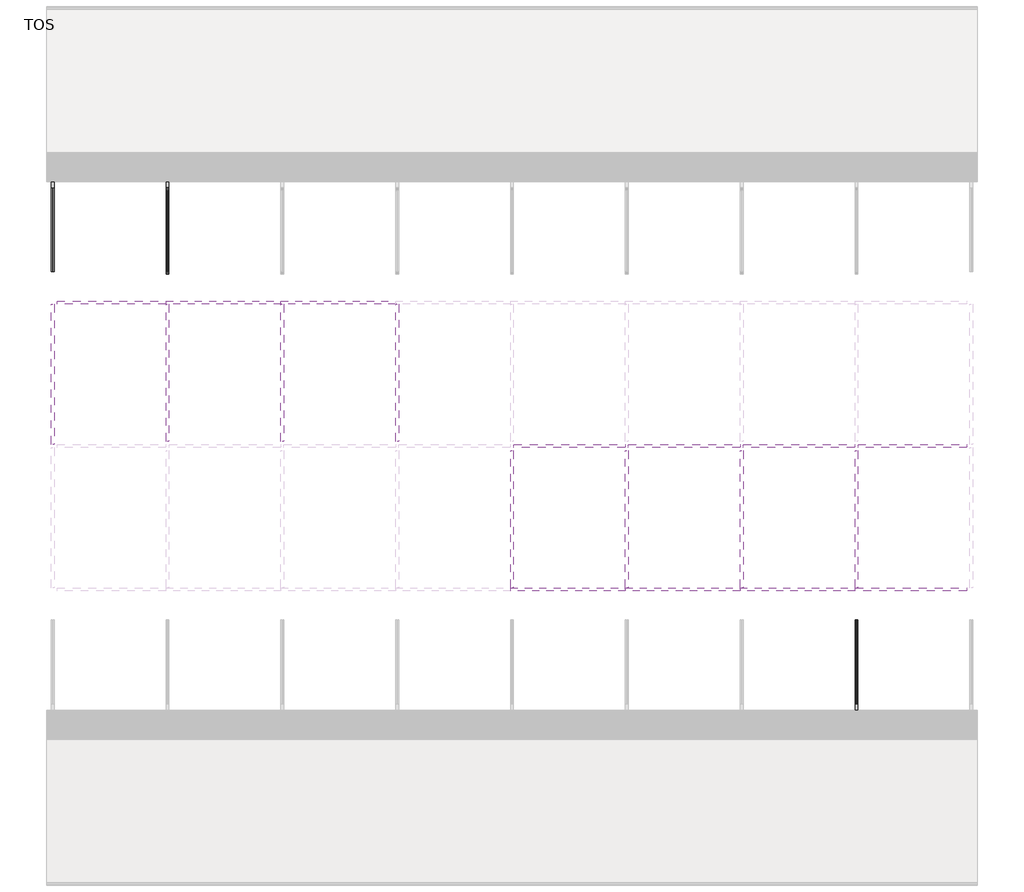
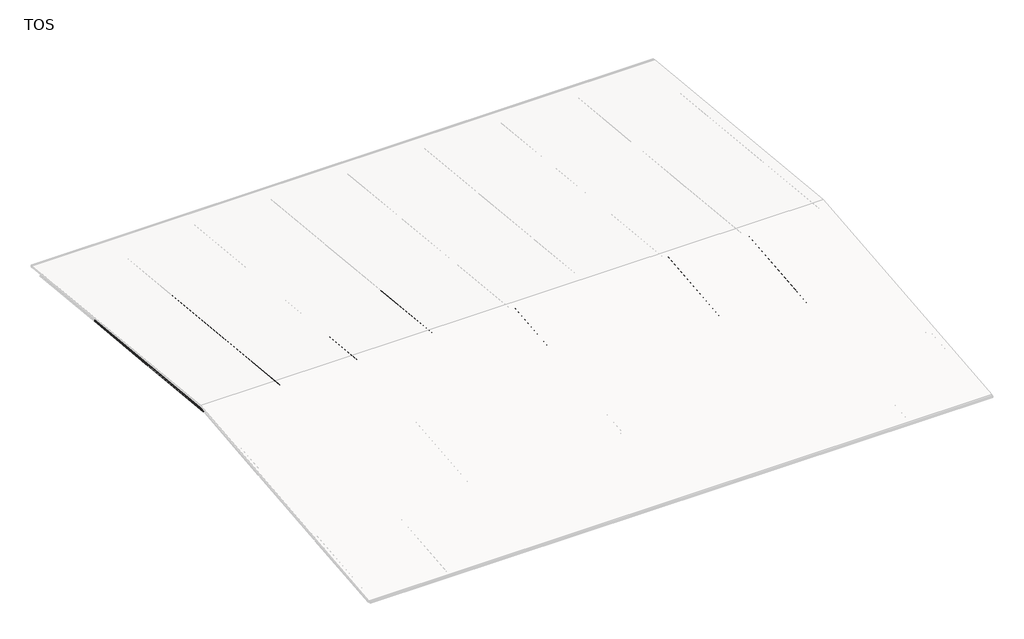
# One storey, part 3 of 5: 22 beams.
"""IFC4 building model written with IfcOpenShell, lengths in millimetres."""

from ifc_helpers import new_model, si_unit, point, frame, frame_2d, origin, place, context, project, spatial, polyline, circle_curve, trimmed, segment, composite_curve, outline, extrude, element, save

model = new_model("IFC4")

# Units and contexts
model_context = context("Model", 3, world=origin())
ifc_project = project(units=[si_unit("LENGTHUNIT", "METRE", prefix="MILLI")], contexts=[model_context])

# Site, building, storey
site = spatial("IfcSite", under=ifc_project)
building = spatial("IfcBuilding", under=site)
storey = spatial("IfcBuildingStorey", under=building, Name="TOS", Elevation=9299.9618634)

# Beams
placement = place(None, origin())
element("IfcBeam", 1, ObjectType="0912_Steel Framing_H-KSD3502 : H_SB_ASB_H-600x200x11x17", at=placement, inside=storey, context=model_context, shape_type="SweptSolid", body=[
    extrude(outline(composite_curve([segment(polyline([(20599.5208589, 10716.9618634), (20599.5208589, 10699.9618634), (20399.5208589, 10699.9618634), (20399.5208589, 10716.9618634), (20472.0208589, 10716.9618634)]), True, "CONTINUOUS"), segment(trimmed(circle_curve(frame_2d((20472.0208589, 10738.9618634)), 22.0), [point((20472.0208589, 10716.9618634))], [point((20494.0208589, 10738.9618634))], True, "CARTESIAN"), True, "CONTINUOUS"), segment(polyline([(20494.0208589, 10738.9618634), (20494.0208589, 11260.9618634)]), True, "CONTINUOUS"), segment(trimmed(circle_curve(frame_2d((20472.0208589, 11260.9618634)), 22.0), [point((20494.0208589, 11260.9618634))], [point((20472.0208589, 11282.9618634))], True, "CARTESIAN"), True, "CONTINUOUS"), segment(polyline([(20472.0208589, 11282.9618634), (20399.5208589, 11282.9618634), (20399.5208589, 11299.9618634), (20599.5208589, 11299.9618634), (20599.5208589, 11282.9618634), (20527.0208589, 11282.9618634)]), True, "CONTINUOUS"), segment(trimmed(circle_curve(frame_2d((20527.0208589, 11260.9618634)), 22.0), [point((20527.0208589, 11282.9618634))], [point((20505.0208589, 11260.9618634))], True, "CARTESIAN"), True, "CONTINUOUS"), segment(polyline([(20505.0208589, 11260.9618634), (20505.0208589, 10738.9618634)]), True, "CONTINUOUS"), segment(trimmed(circle_curve(frame_2d((20527.0208589, 10738.9618634)), 22.0), [point((20505.0208589, 10738.9618634))], [point((20527.0208589, 10716.9618634))], True, "CARTESIAN"), True, "CONTINUOUS"), segment(polyline([(20527.0208589, 10716.9618634), (20599.5208589, 10716.9618634)]), True, "CONTINUOUS")], self_intersect=False)), frame((31900.0, 0.0, 0.0), z_axis=(1.0, 0.0, 0.0), x_axis=(0.0, 1.0, 0.0)), (0.0, 0.0, 1.0), 7987.3),
])
element("IfcBeam", 2, ObjectType="0912_Steel Framing_H-KSD3502 : H_SB_ASB_H-600x200x11x17", at=placement, inside=storey, context=model_context, shape_type="SweptSolid", body=[
    extrude(outline(composite_curve([segment(polyline([(20599.5208589, 10716.9618634), (20599.5208589, 10699.9618634), (20399.5208589, 10699.9618634), (20399.5208589, 10716.9618634), (20472.0208589, 10716.9618634)]), True, "CONTINUOUS"), segment(trimmed(circle_curve(frame_2d((20472.0208589, 10738.9618634)), 22.0), [point((20472.0208589, 10716.9618634))], [point((20494.0208589, 10738.9618634))], True, "CARTESIAN"), True, "CONTINUOUS"), segment(polyline([(20494.0208589, 10738.9618634), (20494.0208589, 11260.9618634)]), True, "CONTINUOUS"), segment(trimmed(circle_curve(frame_2d((20472.0208589, 11260.9618634)), 22.0), [point((20494.0208589, 11260.9618634))], [point((20472.0208589, 11282.9618634))], True, "CARTESIAN"), True, "CONTINUOUS"), segment(polyline([(20472.0208589, 11282.9618634), (20399.5208589, 11282.9618634), (20399.5208589, 11299.9618634), (20599.5208589, 11299.9618634), (20599.5208589, 11282.9618634), (20527.0208589, 11282.9618634)]), True, "CONTINUOUS"), segment(trimmed(circle_curve(frame_2d((20527.0208589, 11260.9618634)), 22.0), [point((20527.0208589, 11282.9618634))], [point((20505.0208589, 11260.9618634))], True, "CARTESIAN"), True, "CONTINUOUS"), segment(polyline([(20505.0208589, 11260.9618634), (20505.0208589, 10738.9618634)]), True, "CONTINUOUS"), segment(trimmed(circle_curve(frame_2d((20527.0208589, 10738.9618634)), 22.0), [point((20505.0208589, 10738.9618634))], [point((20527.0208589, 10716.9618634))], True, "CARTESIAN"), True, "CONTINUOUS"), segment(polyline([(20527.0208589, 10716.9618634), (20599.5208589, 10716.9618634)]), True, "CONTINUOUS")], self_intersect=False)), frame((39900.0, 0.0, 0.0), z_axis=(1.0, 0.0, 0.0), x_axis=(0.0, 1.0, 0.0)), (0.0, 0.0, 1.0), 7987.3),
])
element("IfcBeam", 3, ObjectType="0912_Steel Framing_H-KSD3502 : H_SB_ASB_H-600x200x11x17", at=placement, inside=storey, context=model_context, shape_type="SweptSolid", body=[
    extrude(outline(composite_curve([segment(polyline([(20599.5208589, 10716.9618634), (20599.5208589, 10699.9618634), (20399.5208589, 10699.9618634), (20399.5208589, 10716.9618634), (20472.0208589, 10716.9618634)]), True, "CONTINUOUS"), segment(trimmed(circle_curve(frame_2d((20472.0208589, 10738.9618634)), 22.0), [point((20472.0208589, 10716.9618634))], [point((20494.0208589, 10738.9618634))], True, "CARTESIAN"), True, "CONTINUOUS"), segment(polyline([(20494.0208589, 10738.9618634), (20494.0208589, 11260.9618634)]), True, "CONTINUOUS"), segment(trimmed(circle_curve(frame_2d((20472.0208589, 11260.9618634)), 22.0), [point((20494.0208589, 11260.9618634))], [point((20472.0208589, 11282.9618634))], True, "CARTESIAN"), True, "CONTINUOUS"), segment(polyline([(20472.0208589, 11282.9618634), (20399.5208589, 11282.9618634), (20399.5208589, 11299.9618634), (20599.5208589, 11299.9618634), (20599.5208589, 11282.9618634), (20527.0208589, 11282.9618634)]), True, "CONTINUOUS"), segment(trimmed(circle_curve(frame_2d((20527.0208589, 11260.9618634)), 22.0), [point((20527.0208589, 11282.9618634))], [point((20505.0208589, 11260.9618634))], True, "CARTESIAN"), True, "CONTINUOUS"), segment(polyline([(20505.0208589, 11260.9618634), (20505.0208589, 10738.9618634)]), True, "CONTINUOUS"), segment(trimmed(circle_curve(frame_2d((20527.0208589, 10738.9618634)), 22.0), [point((20505.0208589, 10738.9618634))], [point((20527.0208589, 10716.9618634))], True, "CARTESIAN"), True, "CONTINUOUS"), segment(polyline([(20527.0208589, 10716.9618634), (20599.5208589, 10716.9618634)]), True, "CONTINUOUS")], self_intersect=False)), frame((47900.0, 0.0, 0.0), z_axis=(1.0, 0.0, 0.0), x_axis=(0.0, 1.0, 0.0)), (0.0, 0.0, 1.0), 7987.3),
])
element("IfcBeam", 4, ObjectType="0912_Steel Framing_H-KSD3502 : H_SB_ASB_H-600x200x11x17", at=placement, inside=storey, context=model_context, shape_type="SweptSolid", body=[
    extrude(outline(composite_curve([segment(polyline([(20599.5208589, 10716.9618634), (20599.5208589, 10699.9618634), (20399.5208589, 10699.9618634), (20399.5208589, 10716.9618634), (20472.0208589, 10716.9618634)]), True, "CONTINUOUS"), segment(trimmed(circle_curve(frame_2d((20472.0208589, 10738.9618634)), 22.0), [point((20472.0208589, 10716.9618634))], [point((20494.0208589, 10738.9618634))], True, "CARTESIAN"), True, "CONTINUOUS"), segment(polyline([(20494.0208589, 10738.9618634), (20494.0208589, 11260.9618634)]), True, "CONTINUOUS"), segment(trimmed(circle_curve(frame_2d((20472.0208589, 11260.9618634)), 22.0), [point((20494.0208589, 11260.9618634))], [point((20472.0208589, 11282.9618634))], True, "CARTESIAN"), True, "CONTINUOUS"), segment(polyline([(20472.0208589, 11282.9618634), (20399.5208589, 11282.9618634), (20399.5208589, 11299.9618634), (20599.5208589, 11299.9618634), (20599.5208589, 11282.9618634), (20527.0208589, 11282.9618634)]), True, "CONTINUOUS"), segment(trimmed(circle_curve(frame_2d((20527.0208589, 11260.9618634)), 22.0), [point((20527.0208589, 11282.9618634))], [point((20505.0208589, 11260.9618634))], True, "CARTESIAN"), True, "CONTINUOUS"), segment(polyline([(20505.0208589, 11260.9618634), (20505.0208589, 10738.9618634)]), True, "CONTINUOUS"), segment(trimmed(circle_curve(frame_2d((20527.0208589, 10738.9618634)), 22.0), [point((20505.0208589, 10738.9618634))], [point((20527.0208589, 10716.9618634))], True, "CARTESIAN"), True, "CONTINUOUS"), segment(polyline([(20527.0208589, 10716.9618634), (20599.5208589, 10716.9618634)]), True, "CONTINUOUS")], self_intersect=False)), frame((55900.0, 0.0, 0.0), z_axis=(1.0, 0.0, 0.0), x_axis=(0.0, 1.0, 0.0)), (0.0, 0.0, 1.0), 7781.3),
])
element("IfcBeam", 5, ObjectType="0912_Steel Framing_H-KSD3502 : H_SB_ASB_H-600x200x11x17", at=placement, inside=storey, context=model_context, shape_type="SweptSolid", body=[
    extrude(outline(composite_curve([segment(polyline([(30599.5208589, 11716.9618634), (30599.5208589, 11699.9618634), (30399.5208589, 11699.9618634), (30399.5208589, 11716.9618634), (30472.0208589, 11716.9618634)]), True, "CONTINUOUS"), segment(trimmed(circle_curve(frame_2d((30472.0208589, 11738.9618634)), 22.0), [point((30472.0208589, 11716.9618634))], [point((30494.0208589, 11738.9618634))], True, "CARTESIAN"), True, "CONTINUOUS"), segment(polyline([(30494.0208589, 11738.9618634), (30494.0208589, 12260.9618634)]), True, "CONTINUOUS"), segment(trimmed(circle_curve(frame_2d((30472.0208589, 12260.9618634)), 22.0), [point((30494.0208589, 12260.9618634))], [point((30472.0208589, 12282.9618634))], True, "CARTESIAN"), True, "CONTINUOUS"), segment(polyline([(30472.0208589, 12282.9618634), (30399.5208589, 12282.9618634), (30399.5208589, 12299.9618634), (30599.5208589, 12299.9618634), (30599.5208589, 12282.9618634), (30527.0208589, 12282.9618634)]), True, "CONTINUOUS"), segment(trimmed(circle_curve(frame_2d((30527.0208589, 12260.9618634)), 22.0), [point((30527.0208589, 12282.9618634))], [point((30505.0208589, 12260.9618634))], True, "CARTESIAN"), True, "CONTINUOUS"), segment(polyline([(30505.0208589, 12260.9618634), (30505.0208589, 11738.9618634)]), True, "CONTINUOUS"), segment(trimmed(circle_curve(frame_2d((30527.0208589, 11738.9618634)), 22.0), [point((30505.0208589, 11738.9618634))], [point((30527.0208589, 11716.9618634))], True, "CARTESIAN"), True, "CONTINUOUS"), segment(polyline([(30527.0208589, 11716.9618634), (30599.5208589, 11716.9618634)]), True, "CONTINUOUS")], self_intersect=False)), frame((32113.7, 0.0, 0.0), z_axis=(1.0, 0.0, 0.0), x_axis=(0.0, 1.0, 0.0)), (0.0, 0.0, 1.0), 7772.6),
])
element("IfcBeam", 6, ObjectType="0912_Steel Framing_H-KSD3502 : H_SB_ASB_H-600x200x11x17", at=placement, inside=storey, context=model_context, shape_type="SweptSolid", body=[
    extrude(outline(composite_curve([segment(polyline([(30599.5208589, 11716.9618634), (30599.5208589, 11699.9618634), (30399.5208589, 11699.9618634), (30399.5208589, 11716.9618634), (30472.0208589, 11716.9618634)]), True, "CONTINUOUS"), segment(trimmed(circle_curve(frame_2d((30472.0208589, 11738.9618634)), 22.0), [point((30472.0208589, 11716.9618634))], [point((30494.0208589, 11738.9618634))], True, "CARTESIAN"), True, "CONTINUOUS"), segment(polyline([(30494.0208589, 11738.9618634), (30494.0208589, 12260.9618634)]), True, "CONTINUOUS"), segment(trimmed(circle_curve(frame_2d((30472.0208589, 12260.9618634)), 22.0), [point((30494.0208589, 12260.9618634))], [point((30472.0208589, 12282.9618634))], True, "CARTESIAN"), True, "CONTINUOUS"), segment(polyline([(30472.0208589, 12282.9618634), (30399.5208589, 12282.9618634), (30399.5208589, 12299.9618634), (30599.5208589, 12299.9618634), (30599.5208589, 12282.9618634), (30527.0208589, 12282.9618634)]), True, "CONTINUOUS"), segment(trimmed(circle_curve(frame_2d((30527.0208589, 12260.9618634)), 22.0), [point((30527.0208589, 12282.9618634))], [point((30505.0208589, 12260.9618634))], True, "CARTESIAN"), True, "CONTINUOUS"), segment(polyline([(30505.0208589, 12260.9618634), (30505.0208589, 11738.9618634)]), True, "CONTINUOUS"), segment(trimmed(circle_curve(frame_2d((30527.0208589, 11738.9618634)), 22.0), [point((30505.0208589, 11738.9618634))], [point((30527.0208589, 11716.9618634))], True, "CARTESIAN"), True, "CONTINUOUS"), segment(polyline([(30527.0208589, 11716.9618634), (30599.5208589, 11716.9618634)]), True, "CONTINUOUS")], self_intersect=False)), frame((40113.7, 0.0, 0.0), z_axis=(1.0, 0.0, 0.0), x_axis=(0.0, 1.0, 0.0)), (0.0, 0.0, 1.0), 7772.6),
])
element("IfcBeam", 7, ObjectType="0912_Steel Framing_H-KSD3502 : H_SB_ASB_H-600x200x11x17", at=placement, inside=storey, context=model_context, shape_type="SweptSolid", body=[
    extrude(outline(composite_curve([segment(polyline([(30599.5208589, 11716.9618634), (30599.5208589, 11699.9618634), (30399.5208589, 11699.9618634), (30399.5208589, 11716.9618634), (30472.0208589, 11716.9618634)]), True, "CONTINUOUS"), segment(trimmed(circle_curve(frame_2d((30472.0208589, 11738.9618634)), 22.0), [point((30472.0208589, 11716.9618634))], [point((30494.0208589, 11738.9618634))], True, "CARTESIAN"), True, "CONTINUOUS"), segment(polyline([(30494.0208589, 11738.9618634), (30494.0208589, 12260.9618634)]), True, "CONTINUOUS"), segment(trimmed(circle_curve(frame_2d((30472.0208589, 12260.9618634)), 22.0), [point((30494.0208589, 12260.9618634))], [point((30472.0208589, 12282.9618634))], True, "CARTESIAN"), True, "CONTINUOUS"), segment(polyline([(30472.0208589, 12282.9618634), (30399.5208589, 12282.9618634), (30399.5208589, 12299.9618634), (30599.5208589, 12299.9618634), (30599.5208589, 12282.9618634), (30527.0208589, 12282.9618634)]), True, "CONTINUOUS"), segment(trimmed(circle_curve(frame_2d((30527.0208589, 12260.9618634)), 22.0), [point((30527.0208589, 12282.9618634))], [point((30505.0208589, 12260.9618634))], True, "CARTESIAN"), True, "CONTINUOUS"), segment(polyline([(30505.0208589, 12260.9618634), (30505.0208589, 11738.9618634)]), True, "CONTINUOUS"), segment(trimmed(circle_curve(frame_2d((30527.0208589, 11738.9618634)), 22.0), [point((30505.0208589, 11738.9618634))], [point((30527.0208589, 11716.9618634))], True, "CARTESIAN"), True, "CONTINUOUS"), segment(polyline([(30527.0208589, 11716.9618634), (30599.5208589, 11716.9618634)]), True, "CONTINUOUS")], self_intersect=False)), frame((48113.7, 0.0, 0.0), z_axis=(1.0, 0.0, 0.0), x_axis=(0.0, 1.0, 0.0)), (0.0, 0.0, 1.0), 7772.6),
])
element("IfcBeam", 8, ObjectType="0912_Steel Framing_H-KSD3502 : H_SB_ASB_H-600x200x11x17", at=placement, inside=storey, context=model_context, shape_type="SweptSolid", body=[
    extrude(outline(composite_curve([segment(polyline([(30599.5208589, 11716.9618634), (30599.5208589, 11699.9618634), (30399.5208589, 11699.9618634), (30399.5208589, 11716.9618634), (30472.0208589, 11716.9618634)]), True, "CONTINUOUS"), segment(trimmed(circle_curve(frame_2d((30472.0208589, 11738.9618634)), 22.0), [point((30472.0208589, 11716.9618634))], [point((30494.0208589, 11738.9618634))], True, "CARTESIAN"), True, "CONTINUOUS"), segment(polyline([(30494.0208589, 11738.9618634), (30494.0208589, 12260.9618634)]), True, "CONTINUOUS"), segment(trimmed(circle_curve(frame_2d((30472.0208589, 12260.9618634)), 22.0), [point((30494.0208589, 12260.9618634))], [point((30472.0208589, 12282.9618634))], True, "CARTESIAN"), True, "CONTINUOUS"), segment(polyline([(30472.0208589, 12282.9618634), (30399.5208589, 12282.9618634), (30399.5208589, 12299.9618634), (30599.5208589, 12299.9618634), (30599.5208589, 12282.9618634), (30527.0208589, 12282.9618634)]), True, "CONTINUOUS"), segment(trimmed(circle_curve(frame_2d((30527.0208589, 12260.9618634)), 22.0), [point((30527.0208589, 12282.9618634))], [point((30505.0208589, 12260.9618634))], True, "CARTESIAN"), True, "CONTINUOUS"), segment(polyline([(30505.0208589, 12260.9618634), (30505.0208589, 11738.9618634)]), True, "CONTINUOUS"), segment(trimmed(circle_curve(frame_2d((30527.0208589, 11738.9618634)), 22.0), [point((30505.0208589, 11738.9618634))], [point((30527.0208589, 11716.9618634))], True, "CARTESIAN"), True, "CONTINUOUS"), segment(polyline([(30527.0208589, 11716.9618634), (30599.5208589, 11716.9618634)]), True, "CONTINUOUS")], self_intersect=False)), frame((56113.7, 0.0, 0.0), z_axis=(1.0, 0.0, 0.0), x_axis=(0.0, 1.0, 0.0)), (0.0, 0.0, 1.0), 7567.6),
])
element("IfcBeam", 9, ObjectType="0912_Steel Framing_H-KSD3502 : H_SB_ASB_H-600x200x11x17", at=placement, inside=storey, context=model_context, shape_type="SweptSolid", body=[
    extrude(outline(composite_curve([segment(polyline([(40599.5208589, 10716.9618634), (40599.5208589, 10699.9618634), (40399.5208589, 10699.9618634), (40399.5208589, 10716.9618634), (40472.0208589, 10716.9618634)]), True, "CONTINUOUS"), segment(trimmed(circle_curve(frame_2d((40472.0208589, 10738.9618634)), 22.0), [point((40472.0208589, 10716.9618634))], [point((40494.0208589, 10738.9618634))], True, "CARTESIAN"), True, "CONTINUOUS"), segment(polyline([(40494.0208589, 10738.9618634), (40494.0208589, 11260.9618634)]), True, "CONTINUOUS"), segment(trimmed(circle_curve(frame_2d((40472.0208589, 11260.9618634)), 22.0), [point((40494.0208589, 11260.9618634))], [point((40472.0208589, 11282.9618634))], True, "CARTESIAN"), True, "CONTINUOUS"), segment(polyline([(40472.0208589, 11282.9618634), (40399.5208589, 11282.9618634), (40399.5208589, 11299.9618634), (40599.5208589, 11299.9618634), (40599.5208589, 11282.9618634), (40527.0208589, 11282.9618634)]), True, "CONTINUOUS"), segment(trimmed(circle_curve(frame_2d((40527.0208589, 11260.9618634)), 22.0), [point((40527.0208589, 11282.9618634))], [point((40505.0208589, 11260.9618634))], True, "CARTESIAN"), True, "CONTINUOUS"), segment(polyline([(40505.0208589, 11260.9618634), (40505.0208589, 10738.9618634)]), True, "CONTINUOUS"), segment(trimmed(circle_curve(frame_2d((40527.0208589, 10738.9618634)), 22.0), [point((40505.0208589, 10738.9618634))], [point((40527.0208589, 10716.9618634))], True, "CARTESIAN"), True, "CONTINUOUS"), segment(polyline([(40527.0208589, 10716.9618634), (40599.5208589, 10716.9618634)]), True, "CONTINUOUS")], self_intersect=False)), frame((318.7, 0.0, 0.0), z_axis=(1.0, 0.0, 0.0), x_axis=(0.0, 1.0, 0.0)), (0.0, 0.0, 1.0), 7568.6),
])
element("IfcBeam", 10, ObjectType="0912_Steel Framing_H-KSD3502 : H_SB_ASB_H-600x200x11x17", at=placement, inside=storey, context=model_context, shape_type="SweptSolid", body=[
    extrude(outline(composite_curve([segment(polyline([(40599.5208589, 10716.9618634), (40599.5208589, 10699.9618634), (40399.5208589, 10699.9618634), (40399.5208589, 10716.9618634), (40472.0208589, 10716.9618634)]), True, "CONTINUOUS"), segment(trimmed(circle_curve(frame_2d((40472.0208589, 10738.9618634)), 22.0), [point((40472.0208589, 10716.9618634))], [point((40494.0208589, 10738.9618634))], True, "CARTESIAN"), True, "CONTINUOUS"), segment(polyline([(40494.0208589, 10738.9618634), (40494.0208589, 11260.9618634)]), True, "CONTINUOUS"), segment(trimmed(circle_curve(frame_2d((40472.0208589, 11260.9618634)), 22.0), [point((40494.0208589, 11260.9618634))], [point((40472.0208589, 11282.9618634))], True, "CARTESIAN"), True, "CONTINUOUS"), segment(polyline([(40472.0208589, 11282.9618634), (40399.5208589, 11282.9618634), (40399.5208589, 11299.9618634), (40599.5208589, 11299.9618634), (40599.5208589, 11282.9618634), (40527.0208589, 11282.9618634)]), True, "CONTINUOUS"), segment(trimmed(circle_curve(frame_2d((40527.0208589, 11260.9618634)), 22.0), [point((40527.0208589, 11282.9618634))], [point((40505.0208589, 11260.9618634))], True, "CARTESIAN"), True, "CONTINUOUS"), segment(polyline([(40505.0208589, 11260.9618634), (40505.0208589, 10738.9618634)]), True, "CONTINUOUS"), segment(trimmed(circle_curve(frame_2d((40527.0208589, 10738.9618634)), 22.0), [point((40505.0208589, 10738.9618634))], [point((40527.0208589, 10716.9618634))], True, "CARTESIAN"), True, "CONTINUOUS"), segment(polyline([(40527.0208589, 10716.9618634), (40599.5208589, 10716.9618634)]), True, "CONTINUOUS")], self_intersect=False)), frame((7900.0, 0.0, 0.0), z_axis=(1.0, 0.0, 0.0), x_axis=(0.0, 1.0, 0.0)), (0.0, 0.0, 1.0), 7987.3),
])
element("IfcBeam", 11, ObjectType="0912_Steel Framing_H-KSD3502 : H_SB_ASB_H-600x200x11x17", at=placement, inside=storey, context=model_context, shape_type="SweptSolid", body=[
    extrude(outline(composite_curve([segment(polyline([(40599.5208589, 10716.9618634), (40599.5208589, 10699.9618634), (40399.5208589, 10699.9618634), (40399.5208589, 10716.9618634), (40472.0208589, 10716.9618634)]), True, "CONTINUOUS"), segment(trimmed(circle_curve(frame_2d((40472.0208589, 10738.9618634)), 22.0), [point((40472.0208589, 10716.9618634))], [point((40494.0208589, 10738.9618634))], True, "CARTESIAN"), True, "CONTINUOUS"), segment(polyline([(40494.0208589, 10738.9618634), (40494.0208589, 11260.9618634)]), True, "CONTINUOUS"), segment(trimmed(circle_curve(frame_2d((40472.0208589, 11260.9618634)), 22.0), [point((40494.0208589, 11260.9618634))], [point((40472.0208589, 11282.9618634))], True, "CARTESIAN"), True, "CONTINUOUS"), segment(polyline([(40472.0208589, 11282.9618634), (40399.5208589, 11282.9618634), (40399.5208589, 11299.9618634), (40599.5208589, 11299.9618634), (40599.5208589, 11282.9618634), (40527.0208589, 11282.9618634)]), True, "CONTINUOUS"), segment(trimmed(circle_curve(frame_2d((40527.0208589, 11260.9618634)), 22.0), [point((40527.0208589, 11282.9618634))], [point((40505.0208589, 11260.9618634))], True, "CARTESIAN"), True, "CONTINUOUS"), segment(polyline([(40505.0208589, 11260.9618634), (40505.0208589, 10738.9618634)]), True, "CONTINUOUS"), segment(trimmed(circle_curve(frame_2d((40527.0208589, 10738.9618634)), 22.0), [point((40505.0208589, 10738.9618634))], [point((40527.0208589, 10716.9618634))], True, "CARTESIAN"), True, "CONTINUOUS"), segment(polyline([(40527.0208589, 10716.9618634), (40599.5208589, 10716.9618634)]), True, "CONTINUOUS")], self_intersect=False)), frame((15900.0, 0.0, 0.0), z_axis=(1.0, 0.0, 0.0), x_axis=(0.0, 1.0, 0.0)), (0.0, 0.0, 1.0), 7987.3),
])
element("IfcBeam", 12, ObjectType="0912_Steel Framing_H-KSD3502 : H_SB_ASB_H-600x200x11x17", at=placement, inside=storey, context=model_context, shape_type="SweptSolid", body=[
    extrude(outline(composite_curve([segment(polyline([(-283.0, 100.0), (-283.0, 27.5)]), True, "CONTINUOUS"), segment(trimmed(circle_curve(frame_2d((-261.0, 27.5)), 22.0), [point((-283.0, 27.5))], [point((-261.0, 5.5))], True, "CARTESIAN"), True, "CONTINUOUS"), segment(polyline([(-261.0, 5.5), (261.0, 5.5)]), True, "CONTINUOUS"), segment(trimmed(circle_curve(frame_2d((261.0, 27.5)), 22.0), [point((261.0, 5.5))], [point((283.0000001, 27.5))], True, "CARTESIAN"), True, "CONTINUOUS"), segment(polyline([(283.0000001, 27.5), (283.0000001, 100.0), (300.0, 100.0), (300.0, -100.0), (283.0000001, -100.0), (283.0000001, -27.5)]), True, "CONTINUOUS"), segment(trimmed(circle_curve(frame_2d((261.0, -27.5)), 22.0), [point((283.0000001, -27.5))], [point((261.0, -5.5))], True, "CARTESIAN"), True, "CONTINUOUS"), segment(polyline([(261.0, -5.5), (-261.0, -5.5)]), True, "CONTINUOUS"), segment(trimmed(circle_curve(frame_2d((-261.0, -27.5)), 22.0), [point((-261.0, -5.5))], [point((-283.0, -27.5))], True, "CARTESIAN"), True, "CONTINUOUS"), segment(polyline([(-283.0, -27.5), (-283.0, -100.0), (-299.9999999, -100.0), (-299.9999999, 100.0), (-283.0, 100.0)]), True, "CONTINUOUS")], self_intersect=False)), frame((0.0, 40357.0327709, 11012.7144035), z_axis=(0.0, -0.9950371902099892, 0.09950371902099892), x_axis=(0.0, 0.09950371902099892, 0.9950371902099892)), (0.0, 0.0, 1.0), 9762.4731211),
])
element("IfcBeam", 13, ObjectType="0912_Steel Framing_H-KSD3502 : H_SB_ASB_H-600x200x11x17", at=placement, inside=storey, context=model_context, shape_type="SweptSolid", body=[
    extrude(outline(composite_curve([segment(polyline([(-283.0, 100.0), (-283.0, 27.5)]), True, "CONTINUOUS"), segment(trimmed(circle_curve(frame_2d((-261.0, 27.5)), 22.0), [point((-283.0, 27.5))], [point((-261.0, 5.5))], True, "CARTESIAN"), True, "CONTINUOUS"), segment(polyline([(-261.0, 5.5), (261.0, 5.5)]), True, "CONTINUOUS"), segment(trimmed(circle_curve(frame_2d((261.0, 27.5)), 22.0), [point((261.0, 5.5))], [point((283.0000001, 27.5))], True, "CARTESIAN"), True, "CONTINUOUS"), segment(polyline([(283.0000001, 27.5), (283.0000001, 100.0), (300.0, 100.0), (300.0, -100.0), (283.0000001, -100.0), (283.0000001, -27.5)]), True, "CONTINUOUS"), segment(trimmed(circle_curve(frame_2d((261.0, -27.5)), 22.0), [point((283.0000001, -27.5))], [point((261.0, -5.5))], True, "CARTESIAN"), True, "CONTINUOUS"), segment(polyline([(261.0, -5.5), (-261.0, -5.5)]), True, "CONTINUOUS"), segment(trimmed(circle_curve(frame_2d((-261.0, -27.5)), 22.0), [point((-261.0, -5.5))], [point((-283.0, -27.5))], True, "CARTESIAN"), True, "CONTINUOUS"), segment(polyline([(-283.0, -27.5), (-283.0, -100.0), (-299.9999999, -100.0), (-299.9999999, 100.0), (-283.0, 100.0)]), True, "CONTINUOUS")], self_intersect=False)), frame((0.0, 50357.0327709, 10012.7144035), z_axis=(0.0, -0.9950371902099892, 0.09950371902099896), x_axis=(0.0, 0.09950371902099896, 0.9950371902099892)), (0.0, 0.0, 1.0), 9762.4731211),
])
element("IfcBeam", 14, ObjectType="0912_Steel Framing_H-KSD3502 : H_SB_ASB_H-600x200x11x17", at=placement, inside=storey, context=model_context, shape_type="SweptSolid", body=[
    extrude(outline(composite_curve([segment(polyline([(-283.0, 100.0), (-283.0, 27.5)]), True, "CONTINUOUS"), segment(trimmed(circle_curve(frame_2d((-261.0, 27.5)), 22.0), [point((-283.0, 27.5))], [point((-261.0, 5.5))], True, "CARTESIAN"), True, "CONTINUOUS"), segment(polyline([(-261.0, 5.5), (261.0, 5.5)]), True, "CONTINUOUS"), segment(trimmed(circle_curve(frame_2d((261.0, 27.5)), 22.0), [point((261.0, 5.5))], [point((283.0000001, 27.5))], True, "CARTESIAN"), True, "CONTINUOUS"), segment(polyline([(283.0000001, 27.5), (283.0000001, 100.0), (300.0, 100.0), (300.0, -100.0), (283.0000001, -100.0), (283.0000001, -27.5)]), True, "CONTINUOUS"), segment(trimmed(circle_curve(frame_2d((261.0, -27.5)), 22.0), [point((283.0000001, -27.5))], [point((261.0, -5.5))], True, "CARTESIAN"), True, "CONTINUOUS"), segment(polyline([(261.0, -5.5), (-261.0, -5.5)]), True, "CONTINUOUS"), segment(trimmed(circle_curve(frame_2d((-261.0, -27.5)), 22.0), [point((-261.0, -5.5))], [point((-283.0, -27.5))], True, "CARTESIAN"), True, "CONTINUOUS"), segment(polyline([(-283.0, -27.5), (-283.0, -100.0), (-299.9999999, -100.0), (-299.9999999, 100.0), (-283.0, 100.0)]), True, "CONTINUOUS")], self_intersect=False)), frame((8000.0, 40358.0228699, 11012.6153936), z_axis=(0.0, -0.9950371902099892, 0.09950371902099896), x_axis=(0.0, 0.09950371902099896, 0.9950371902099892)), (0.0, 0.0, 1.0), 9557.4457081),
])
element("IfcBeam", 15, ObjectType="0912_Steel Framing_H-KSD3502 : H_SB_ASB_H-600x200x11x17", at=placement, inside=storey, context=model_context, shape_type="SweptSolid", body=[
    extrude(outline(composite_curve([segment(polyline([(-283.0, 100.0), (-283.0, 27.5)]), True, "CONTINUOUS"), segment(trimmed(circle_curve(frame_2d((-261.0, 27.5)), 22.0), [point((-283.0, 27.5))], [point((-261.0, 5.5))], True, "CARTESIAN"), True, "CONTINUOUS"), segment(polyline([(-261.0, 5.5), (261.0, 5.5)]), True, "CONTINUOUS"), segment(trimmed(circle_curve(frame_2d((261.0, 27.5)), 22.0), [point((261.0, 5.5))], [point((283.0000001, 27.5))], True, "CARTESIAN"), True, "CONTINUOUS"), segment(polyline([(283.0000001, 27.5), (283.0000001, 100.0), (300.0, 100.0), (300.0, -100.0), (283.0000001, -100.0), (283.0000001, -27.5)]), True, "CONTINUOUS"), segment(trimmed(circle_curve(frame_2d((261.0, -27.5)), 22.0), [point((283.0000001, -27.5))], [point((261.0, -5.5))], True, "CARTESIAN"), True, "CONTINUOUS"), segment(polyline([(261.0, -5.5), (-261.0, -5.5)]), True, "CONTINUOUS"), segment(trimmed(circle_curve(frame_2d((-261.0, -27.5)), 22.0), [point((-261.0, -5.5))], [point((-283.0, -27.5))], True, "CARTESIAN"), True, "CONTINUOUS"), segment(polyline([(-283.0, -27.5), (-283.0, -100.0), (-299.9999999, -100.0), (-299.9999999, 100.0), (-283.0, 100.0)]), True, "CONTINUOUS")], self_intersect=False)), frame((8000.0, 50358.0228699, 10012.6153936), z_axis=(0.0, -0.9950371902099892, 0.09950371902099896), x_axis=(0.0, 0.09950371902099896, 0.9950371902099892)), (0.0, 0.0, 1.0), 9765.7659517),
])
element("IfcBeam", 16, ObjectType="0912_Steel Framing_H-KSD3502 : H_SB_ASB_H-600x200x11x17", at=placement, inside=storey, context=model_context, shape_type="SweptSolid", body=[
    extrude(outline(composite_curve([segment(polyline([(-283.0, 100.0), (-283.0, 27.5)]), True, "CONTINUOUS"), segment(trimmed(circle_curve(frame_2d((-261.0, 27.5)), 22.0), [point((-283.0, 27.5))], [point((-261.0, 5.5))], True, "CARTESIAN"), True, "CONTINUOUS"), segment(polyline([(-261.0, 5.5), (261.0, 5.5)]), True, "CONTINUOUS"), segment(trimmed(circle_curve(frame_2d((261.0, 27.5)), 22.0), [point((261.0, 5.5))], [point((283.0000001, 27.5))], True, "CARTESIAN"), True, "CONTINUOUS"), segment(polyline([(283.0000001, 27.5), (283.0000001, 100.0), (300.0, 100.0), (300.0, -100.0), (283.0000001, -100.0), (283.0000001, -27.5)]), True, "CONTINUOUS"), segment(trimmed(circle_curve(frame_2d((261.0, -27.5)), 22.0), [point((283.0000001, -27.5))], [point((261.0, -5.5))], True, "CARTESIAN"), True, "CONTINUOUS"), segment(polyline([(261.0, -5.5), (-261.0, -5.5)]), True, "CONTINUOUS"), segment(trimmed(circle_curve(frame_2d((-261.0, -27.5)), 22.0), [point((-261.0, -5.5))], [point((-283.0, -27.5))], True, "CARTESIAN"), True, "CONTINUOUS"), segment(polyline([(-283.0, -27.5), (-283.0, -100.0), (-299.9999999, -100.0), (-299.9999999, 100.0), (-283.0, 100.0)]), True, "CONTINUOUS")], self_intersect=False)), frame((16000.0, 40358.0228699, 11012.6153936), z_axis=(0.0, -0.9950371902099892, 0.09950371902099896), x_axis=(0.0, 0.09950371902099896, 0.9950371902099892)), (0.0, 0.0, 1.0), 9557.4457081),
])
element("IfcBeam", 17, ObjectType="0912_Steel Framing_H-KSD3502 : H_SB_ASB_H-600x200x11x17", at=placement, inside=storey, context=model_context, shape_type="SweptSolid", body=[
    extrude(outline(composite_curve([segment(polyline([(-283.0, 100.0), (-283.0, 27.5)]), True, "CONTINUOUS"), segment(trimmed(circle_curve(frame_2d((-261.0, 27.5)), 22.0), [point((-283.0, 27.5))], [point((-261.0, 5.5))], True, "CARTESIAN"), True, "CONTINUOUS"), segment(polyline([(-261.0, 5.5), (261.0, 5.5)]), True, "CONTINUOUS"), segment(trimmed(circle_curve(frame_2d((261.0, 27.5)), 22.0), [point((261.0, 5.5))], [point((283.0000001, 27.5))], True, "CARTESIAN"), True, "CONTINUOUS"), segment(polyline([(283.0000001, 27.5), (283.0000001, 100.0), (300.0, 100.0), (300.0, -100.0), (283.0000001, -100.0), (283.0000001, -27.5)]), True, "CONTINUOUS"), segment(trimmed(circle_curve(frame_2d((261.0, -27.5)), 22.0), [point((283.0000001, -27.5))], [point((261.0, -5.5))], True, "CARTESIAN"), True, "CONTINUOUS"), segment(polyline([(261.0, -5.5), (-261.0, -5.5)]), True, "CONTINUOUS"), segment(trimmed(circle_curve(frame_2d((-261.0, -27.5)), 22.0), [point((-261.0, -5.5))], [point((-283.0, -27.5))], True, "CARTESIAN"), True, "CONTINUOUS"), segment(polyline([(-283.0, -27.5), (-283.0, -100.0), (-299.9999999, -100.0), (-299.9999999, 100.0), (-283.0, 100.0)]), True, "CONTINUOUS")], self_intersect=False)), frame((24000.0, 40358.0228699, 11012.6153936), z_axis=(0.0, -0.9950371902099892, 0.09950371902099892), x_axis=(0.0, 0.09950371902099892, 0.9950371902099892)), (0.0, 0.0, 1.0), 9557.4457081),
])
element("IfcBeam", 18, ObjectType="0912_Steel Framing_H-KSD3502 : H_SB_ASB_H-600x200x11x17", at=placement, inside=storey, context=model_context, shape_type="SweptSolid", body=[
    extrude(outline(composite_curve([segment(polyline([(-283.0, -100.0), (-299.9999999, -100.0), (-299.9999999, 100.0), (-283.0, 100.0), (-283.0, 27.5)]), True, "CONTINUOUS"), segment(trimmed(circle_curve(frame_2d((-261.0, 27.5)), 22.0), [point((-283.0, 27.5))], [point((-261.0, 5.5))], True, "CARTESIAN"), True, "CONTINUOUS"), segment(polyline([(-261.0, 5.5), (261.0000001, 5.5)]), True, "CONTINUOUS"), segment(trimmed(circle_curve(frame_2d((261.0000001, 27.5)), 22.0), [point((261.0000001, 5.5))], [point((283.0000001, 27.5))], True, "CARTESIAN"), True, "CONTINUOUS"), segment(polyline([(283.0000001, 27.5), (283.0000001, 100.0), (300.0, 100.0), (300.0, -100.0), (283.0000001, -100.0), (283.0000001, -27.5)]), True, "CONTINUOUS"), segment(trimmed(circle_curve(frame_2d((261.0000001, -27.5)), 22.0), [point((283.0000001, -27.5))], [point((261.0000001, -5.5))], True, "CARTESIAN"), True, "CONTINUOUS"), segment(polyline([(261.0000001, -5.5), (-261.0, -5.5)]), True, "CONTINUOUS"), segment(trimmed(circle_curve(frame_2d((-261.0, -27.5)), 22.0), [point((-261.0, -5.5))], [point((-283.0, -27.5))], True, "CARTESIAN"), True, "CONTINUOUS"), segment(polyline([(-283.0, -27.5), (-283.0, -100.0)]), True, "CONTINUOUS")], self_intersect=False)), frame((32000.0, 20641.0188479, 11012.6153936), z_axis=(0.0, 0.9950371902099892, 0.09950371902099887), x_axis=(0.0, -0.09950371902099887, 0.9950371902099892)), (0.0, 0.0, 1.0), 9557.4457081),
])
element("IfcBeam", 19, ObjectType="0912_Steel Framing_H-KSD3502 : H_SB_ASB_H-600x200x11x17", at=placement, inside=storey, context=model_context, shape_type="SweptSolid", body=[
    extrude(outline(composite_curve([segment(polyline([(-283.0, -100.0), (-299.9999999, -100.0), (-299.9999999, 100.0), (-283.0, 100.0), (-283.0, 27.5)]), True, "CONTINUOUS"), segment(trimmed(circle_curve(frame_2d((-261.0, 27.5)), 22.0), [point((-283.0, 27.5))], [point((-261.0, 5.5))], True, "CARTESIAN"), True, "CONTINUOUS"), segment(polyline([(-261.0, 5.5), (261.0000001, 5.5)]), True, "CONTINUOUS"), segment(trimmed(circle_curve(frame_2d((261.0000001, 27.5)), 22.0), [point((261.0000001, 5.5))], [point((283.0000001, 27.5))], True, "CARTESIAN"), True, "CONTINUOUS"), segment(polyline([(283.0000001, 27.5), (283.0000001, 100.0), (300.0, 100.0), (300.0, -100.0), (283.0000001, -100.0), (283.0000001, -27.5)]), True, "CONTINUOUS"), segment(trimmed(circle_curve(frame_2d((261.0000001, -27.5)), 22.0), [point((283.0000001, -27.5))], [point((261.0000001, -5.5))], True, "CARTESIAN"), True, "CONTINUOUS"), segment(polyline([(261.0000001, -5.5), (-261.0, -5.5)]), True, "CONTINUOUS"), segment(trimmed(circle_curve(frame_2d((-261.0, -27.5)), 22.0), [point((-261.0, -5.5))], [point((-283.0, -27.5))], True, "CARTESIAN"), True, "CONTINUOUS"), segment(polyline([(-283.0, -27.5), (-283.0, -100.0)]), True, "CONTINUOUS")], self_intersect=False)), frame((40000.0, 20641.0188479, 11012.6153936), z_axis=(0.0, 0.9950371902099892, 0.09950371902099887), x_axis=(0.0, -0.09950371902099887, 0.9950371902099892)), (0.0, 0.0, 1.0), 9557.4457081),
])
element("IfcBeam", 20, ObjectType="0912_Steel Framing_H-KSD3502 : H_SB_ASB_H-600x200x11x17", at=placement, inside=storey, context=model_context, shape_type="SweptSolid", body=[
    extrude(outline(composite_curve([segment(polyline([(-283.0, -100.0), (-299.9999999, -100.0), (-299.9999999, 100.0), (-283.0, 100.0), (-283.0, 27.5)]), True, "CONTINUOUS"), segment(trimmed(circle_curve(frame_2d((-261.0, 27.5)), 22.0), [point((-283.0, 27.5))], [point((-261.0, 5.5))], True, "CARTESIAN"), True, "CONTINUOUS"), segment(polyline([(-261.0, 5.5), (261.0000001, 5.5)]), True, "CONTINUOUS"), segment(trimmed(circle_curve(frame_2d((261.0000001, 27.5)), 22.0), [point((261.0000001, 5.5))], [point((283.0000001, 27.5))], True, "CARTESIAN"), True, "CONTINUOUS"), segment(polyline([(283.0000001, 27.5), (283.0000001, 100.0), (300.0, 100.0), (300.0, -100.0), (283.0000001, -100.0), (283.0000001, -27.5)]), True, "CONTINUOUS"), segment(trimmed(circle_curve(frame_2d((261.0000001, -27.5)), 22.0), [point((283.0000001, -27.5))], [point((261.0000001, -5.5))], True, "CARTESIAN"), True, "CONTINUOUS"), segment(polyline([(261.0000001, -5.5), (-261.0, -5.5)]), True, "CONTINUOUS"), segment(trimmed(circle_curve(frame_2d((-261.0, -27.5)), 22.0), [point((-261.0, -5.5))], [point((-283.0, -27.5))], True, "CARTESIAN"), True, "CONTINUOUS"), segment(polyline([(-283.0, -27.5), (-283.0, -100.0)]), True, "CONTINUOUS")], self_intersect=False)), frame((48000.0, 20641.0188479, 11012.6153936), z_axis=(0.0, 0.9950371902099892, 0.09950371902099887), x_axis=(0.0, -0.09950371902099887, 0.9950371902099892)), (0.0, 0.0, 1.0), 9557.4457081),
])
element("IfcBeam", 21, ObjectType="0912_Steel Framing_H-KSD3502 : H_SB_ASB_H-600x200x11x17", at=placement, inside=storey, context=model_context, shape_type="SweptSolid", body=[
    extrude(outline(composite_curve([segment(polyline([(-283.0, -100.0), (-299.9999999, -100.0), (-299.9999999, 100.0), (-283.0, 100.0), (-283.0, 27.5)]), True, "CONTINUOUS"), segment(trimmed(circle_curve(frame_2d((-261.0, 27.5)), 22.0), [point((-283.0, 27.5))], [point((-261.0, 5.5))], True, "CARTESIAN"), True, "CONTINUOUS"), segment(polyline([(-261.0, 5.5), (261.0000001, 5.5)]), True, "CONTINUOUS"), segment(trimmed(circle_curve(frame_2d((261.0000001, 27.5)), 22.0), [point((261.0000001, 5.5))], [point((283.0000001, 27.5))], True, "CARTESIAN"), True, "CONTINUOUS"), segment(polyline([(283.0000001, 27.5), (283.0000001, 100.0), (300.0, 100.0), (300.0, -100.0), (283.0000001, -100.0), (283.0000001, -27.5)]), True, "CONTINUOUS"), segment(trimmed(circle_curve(frame_2d((261.0000001, -27.5)), 22.0), [point((283.0000001, -27.5))], [point((261.0000001, -5.5))], True, "CARTESIAN"), True, "CONTINUOUS"), segment(polyline([(261.0000001, -5.5), (-261.0, -5.5)]), True, "CONTINUOUS"), segment(trimmed(circle_curve(frame_2d((-261.0, -27.5)), 22.0), [point((-261.0, -5.5))], [point((-283.0, -27.5))], True, "CARTESIAN"), True, "CONTINUOUS"), segment(polyline([(-283.0, -27.5), (-283.0, -100.0)]), True, "CONTINUOUS")], self_intersect=False)), frame((56000.0, 10641.0188479, 10012.6153936), z_axis=(0.0, 0.9950371902099892, 0.09950371902099894), x_axis=(0.0, -0.09950371902099894, 0.9950371902099892)), (0.0, 0.0, 1.0), 9765.7659517),
])
element("IfcBeam", 22, ObjectType="0912_Steel Framing_H-KSD3502 : H_SB_ASB_H-600x200x11x17", at=placement, inside=storey, context=model_context, shape_type="SweptSolid", body=[
    extrude(outline(composite_curve([segment(polyline([(-283.0, -100.0), (-299.9999999, -100.0), (-299.9999999, 100.0), (-283.0, 100.0), (-283.0, 27.5)]), True, "CONTINUOUS"), segment(trimmed(circle_curve(frame_2d((-261.0, 27.5)), 22.0), [point((-283.0, 27.5))], [point((-261.0, 5.5))], True, "CARTESIAN"), True, "CONTINUOUS"), segment(polyline([(-261.0, 5.5), (261.0000001, 5.5)]), True, "CONTINUOUS"), segment(trimmed(circle_curve(frame_2d((261.0000001, 27.5)), 22.0), [point((261.0000001, 5.5))], [point((283.0000001, 27.5))], True, "CARTESIAN"), True, "CONTINUOUS"), segment(polyline([(283.0000001, 27.5), (283.0000001, 100.0), (300.0, 100.0), (300.0, -100.0), (283.0000001, -100.0), (283.0000001, -27.5)]), True, "CONTINUOUS"), segment(trimmed(circle_curve(frame_2d((261.0000001, -27.5)), 22.0), [point((283.0000001, -27.5))], [point((261.0000001, -5.5))], True, "CARTESIAN"), True, "CONTINUOUS"), segment(polyline([(261.0000001, -5.5), (-261.0, -5.5)]), True, "CONTINUOUS"), segment(trimmed(circle_curve(frame_2d((-261.0, -27.5)), 22.0), [point((-261.0, -5.5))], [point((-283.0, -27.5))], True, "CARTESIAN"), True, "CONTINUOUS"), segment(polyline([(-283.0, -27.5), (-283.0, -100.0)]), True, "CONTINUOUS")], self_intersect=False)), frame((56000.0, 20641.0188479, 11012.6153936), z_axis=(0.0, 0.9950371902099892, 0.09950371902099896), x_axis=(0.0, -0.09950371902099896, 0.9950371902099892)), (0.0, 0.0, 1.0), 9557.4457081),
])

save(model, "model.ifc")

# Revit data of these elements
# Type "0912_Steel Framing_H-KSD3502 : H_SB_ASB_H-600x200x11x17"
#   Width = 20.0 cm
#   Web Thickness = 1.1 cm
#   Web Fillet = 2.2 cm
#   Warping Constant = 1930000.0 cm⁶
#   W = 0
#   Torsional Moment of Inertia = 91.3724 cm⁴
#   Section Area = 134.4 cm²
#   Plastic Modulus weak axis = 361.0 cm³
#   Plastic Modulus strong axis = 2980.0 cm³
#   Perimeter = 1.94 m²/m
#   Nominal Weight = 106.00 kgf/m
#   Moment of Inertia weak axis = 2280.00 cm⁴
#   Moment of Inertia strong axis = 77600.00 cm⁴
#   Height = 60.0 cm
#   Flange Thickness = 1.7 cm
#   Elastic Modulus weak axis = 228.0 cm³
#   Elastic Modulus strong axis = 2590.0 cm³
#   Centroid Vertical = 30.0 cm
#   Centroid Horizontal = 10.0 cm
#   Ix = 776000000
#   Length [instance default] = 1524 mm
#   Zx = 2980000
#   b = 200 mm
#   h = 600 mm
#   r = 22 mm
#   s = 11 mm
#   t = 17 mm
#   A = 0.01344 m²
#   Structural Material [instance default] = Steel, 45-345
#   Assembly Code = ""
# Elements 1, 2, 3, 4, 5, 6, 7, 8, 9, 10, 11, 12, 13, 14, 15, 16, 17, 18, 19, 20, 21, 22 (IfcBeam, "0912_Steel Framing_H-KSD3502 : H_SB_ASB_H-600x200x11x17")
#   Comments = ""
#   Phase Created = New Construction
#   Materials on its faces: "Steel, 45-345"
# Materials
#   "Steel, 45-345": class "Metal", colour RGB 189 187 185, transparency 0, Description = "Steel 345 MPa", Cost = 0
